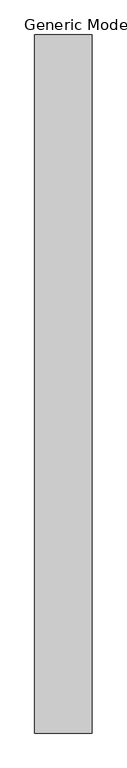
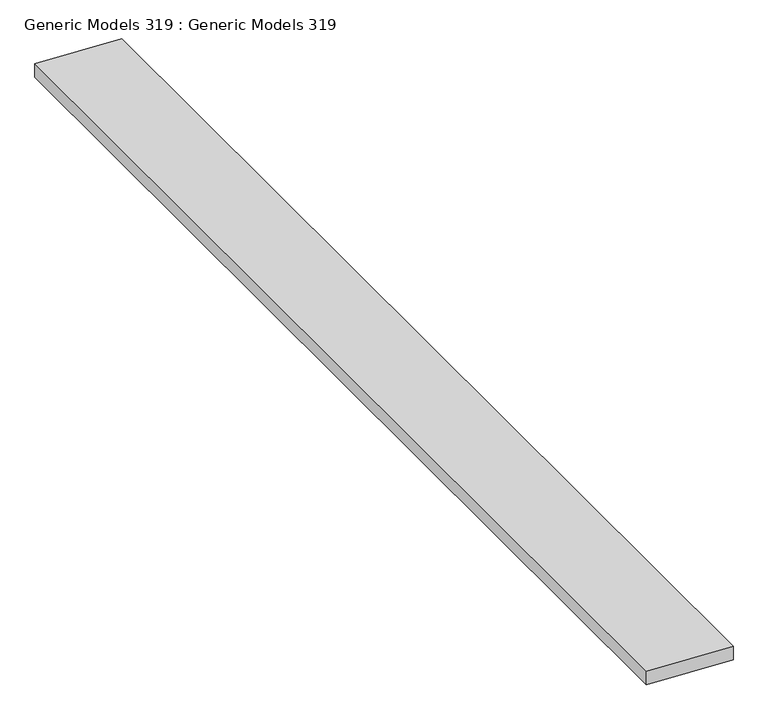
"""IFC4 building model written with IfcOpenShell, lengths in millimetres: proxy geometry, Generic Models 319 : Generic Models 319."""

from ifc_helpers import new_model, si_unit, frame, origin, place, context, project, spatial, polyline, outline, extrude, source, transform, mapped, element, save


def generic_models_319_generic_models_319_50e36bff(model_context):
    return source(origin(), model_context, "Body", "SweptSolid", [
        extrude(outline(polyline([(123747.1569375, 8750.1263705), (123594.5880456, 8750.1263705), (123551.5271081, 9664.5263705), (123704.096, 9664.5263705), (123747.1569375, 8750.1263705)])), frame((0.0, -4109.6428838, 0.0), z_axis=(0.0, 1.0, 0.0), x_axis=(0.0, 0.0, 1.0)), (0.0, 0.0, 1.0), 11163.91985),
    ])


if __name__ == "__main__":
    model = new_model("IFC4")
    model_context = context("Model", 3, world=origin())
    ifc_project = project(units=[si_unit("LENGTHUNIT", "METRE", prefix="MILLI")], contexts=[model_context])
    site = spatial("IfcSite", under=ifc_project)
    building = spatial("IfcBuilding", under=site)
    placement = place(None, origin())
    generic_models_319_generic_models_319_shape = generic_models_319_generic_models_319_50e36bff(model_context)
    element("IfcBuildingElementProxy", 1, Name="Generic Models 319 : Generic Models 319", ObjectType="Generic Models 319 : Generic Models 319", at=placement, inside=building, context=model_context, shape_type="MappedRepresentation", body=[
        mapped(generic_models_319_generic_models_319_shape, transform((0.0, 0.0, 0.0), x_axis=(1.0, 0.0, 0.0), y_axis=(0.0, 1.0, 0.0), z_axis=(0.0, 0.0, 1.0))),
    ])
    save(model, "model.ifc")

# Revit data of these elements
# Element 1 (IfcBuildingElementProxy, "Generic Models 319 : Generic Models 319")
#   Materials on its faces: "_6\" CONCRETE PAVERS W/ WIRE MESH"
# Materials
#   "_6\" CONCRETE PAVERS W/ WIRE MESH": class "Generic", colour RGB 191 191 191, transparency 0, Cost = 0
